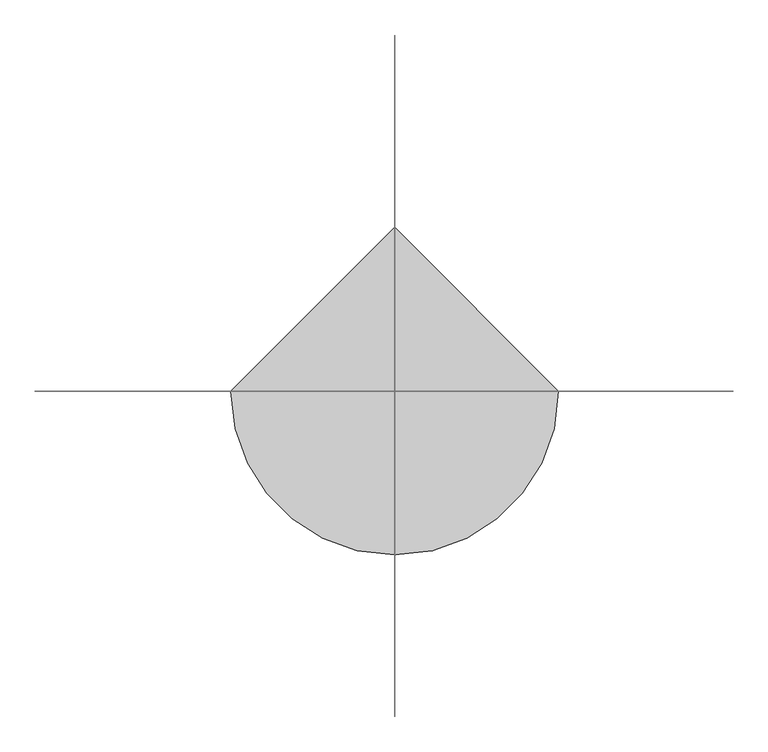
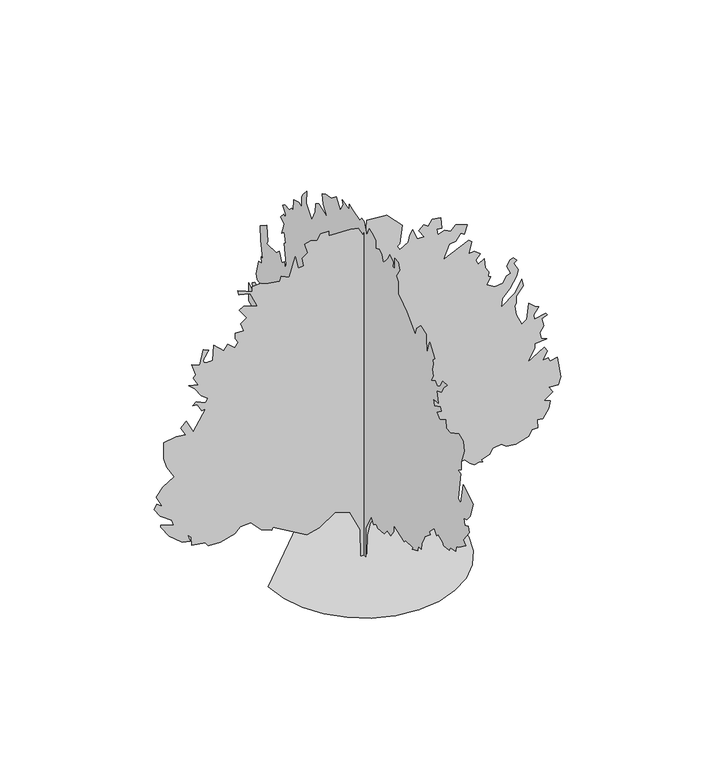
"""IFC4 building model written with IfcOpenShell, lengths in millimetres: proxy geometry, daphne 26070 : daphne 26070."""

import ifcopenshell
import ifcopenshell.guid

model = None  # the IFC model being written
_history = None  # IfcOwnerHistory: only IFC2X3 demands one
_inside = {}  # id of a spatial element -> (the spatial element, [elements in it])
_under = {}  # id of a project, library or spatial element -> (it, [spatial elements below it])
_declared = {}  # id of a project -> (the project, [libraries it declares])
_typed = {}  # id of a type object -> (the type object, [elements of that type])
_made_of = {}  # id of a material, layer set ... -> (it, [elements and type objects made of it])


def new_model(schema):
    """Start an empty IFC model of exactly this schema.

    Asked for "IFC4X3", IfcOpenShell would pick the latest addendum, in which some entities
    have other attributes; the version numbers below select the first issue.
    IFC2X3 requires an IfcOwnerHistory on every rooted entity: one is made here for all.
    """
    global model, _history
    if schema == "IFC4X3":
        model = ifcopenshell.file(schema_version=(4, 3, 0, 0))
    else:
        model = ifcopenshell.file(schema=schema)
    _inside.clear()
    _under.clear()
    _declared.clear()
    _typed.clear()
    _made_of.clear()
    _history = None
    if model.schema == "IFC2X3":
        org = make("IfcOrganization", Name="unknown")
        user = make(
            "IfcPersonAndOrganization",
            ThePerson=make("IfcPerson", FamilyName="unknown"),
            TheOrganization=org,
        )
        app = make(
            "IfcApplication",
            ApplicationDeveloper=org,
            Version="unknown",
            ApplicationFullName="unknown",
            ApplicationIdentifier="unknown",
        )
        _history = make(
            "IfcOwnerHistory",
            OwningUser=user,
            OwningApplication=app,
            ChangeAction="ADDED",
            CreationDate=0,
        )
    return model


def make(cls, **values):
    """One entity of the class cls with the attributes given. An attribute that is None is left unset."""
    return model.create_entity(
        cls, **{name: value for name, value in values.items() if value is not None}
    )


def rooted(cls, **values):
    """An entity with a GlobalId (a new one), such as an element, a storey or a relation."""
    return make(cls, GlobalId=ifcopenshell.guid.new(), OwnerHistory=_history, **values)


def si_unit(unit_type, name, prefix=None):
    """IfcSIUnit, for example si_unit("LENGTHUNIT", "METRE", prefix="MILLI")."""
    return make("IfcSIUnit", UnitType=unit_type, Prefix=prefix, Name=name)


def assignment(units):
    """IfcUnitAssignment: the units of a project."""
    return None if units is None else make("IfcUnitAssignment", Units=units)


def point(xyz):
    """IfcCartesianPoint."""
    return None if xyz is None else make("IfcCartesianPoint", Coordinates=xyz)


def direction(xyz):
    """IfcDirection."""
    return None if xyz is None else make("IfcDirection", DirectionRatios=xyz)


def frame(location, z_axis=None, x_axis=None):
    """IfcAxis2Placement3D, a coordinate frame: its origin and axes. An axis left out is left unset."""
    return make(
        "IfcAxis2Placement3D",
        Location=point(location),
        Axis=direction(z_axis),
        RefDirection=direction(x_axis),
    )


def origin():
    """The frame at (0, 0, 0) with its axes left unset."""
    return frame((0.0, 0.0, 0.0))


def place(relative_to, where):
    """IfcLocalPlacement: puts the frame where relative to a parent placement (None: the world)."""
    return make(
        "IfcLocalPlacement", PlacementRelTo=relative_to, RelativePlacement=where
    )


def context(
    kind, dimensions, precision=None, world=None, true_north=None, identifier=None
):
    """IfcGeometricRepresentationContext, for example the 3D "Model" context."""
    return make(
        "IfcGeometricRepresentationContext",
        ContextIdentifier=identifier,
        ContextType=kind,
        CoordinateSpaceDimension=dimensions,
        Precision=precision,
        WorldCoordinateSystem=world,
        TrueNorth=true_north,
    )


def project(units=None, contexts=None):
    """IfcProject with its units and contexts."""
    return rooted(
        "IfcProject",
        Name="project",
        RepresentationContexts=contexts,
        UnitsInContext=assignment(units),
    )


def spatial(cls, under=None, at=None, **own):
    """A site, building, storey or space (cls), placed at a placement, below another one or the project."""
    s = rooted(cls, ObjectPlacement=at, **own)
    if under is not None:
        _under.setdefault(under.id(), (under, []))[1].append(s)
    return s


def point_list(points):
    """IfcCartesianPointList2D or 3D."""
    cls = (
        "IfcCartesianPointList2D" if len(points[0]) == 2 else "IfcCartesianPointList3D"
    )
    return make(cls, CoordList=points)


def triangles(points, corners, closed=None, point_numbers=None):
    """IfcTriangulatedFaceSet: each triangle names its three corners, points numbered from 1."""
    return make(
        "IfcTriangulatedFaceSet",
        Coordinates=point_list(points),
        Closed=closed,
        CoordIndex=corners,
        PnIndex=point_numbers,
    )


def shape(context_of_items, identifier, shape_type, items):
    """IfcShapeRepresentation: the items that make up one representation, for example the "Body"."""
    return make(
        "IfcShapeRepresentation",
        ContextOfItems=context_of_items,
        RepresentationIdentifier=identifier,
        RepresentationType=shape_type,
        Items=items,
    )


def source(mapping_origin, context_of_items, identifier, shape_type, items):
    """IfcRepresentationMap: a shape defined once, which mapped items show again and again."""
    return make(
        "IfcRepresentationMap",
        MappingOrigin=mapping_origin,
        MappedRepresentation=shape(context_of_items, identifier, shape_type, items),
    )


def transform(
    local_origin,
    x_axis=None,
    y_axis=None,
    z_axis=None,
    scale=None,
    scale2=None,
    scale3=None,
    uniform=True,
):
    """IfcCartesianTransformationOperator3D, or its non-uniform kind. x_axis, y_axis, z_axis: its Axis1, 2, 3."""
    if uniform:
        return make(
            "IfcCartesianTransformationOperator3D",
            Axis1=direction(x_axis),
            Axis2=direction(y_axis),
            LocalOrigin=point(local_origin),
            Scale=scale,
            Axis3=direction(z_axis),
        )
    return make(
        "IfcCartesianTransformationOperator3DnonUniform",
        Axis1=direction(x_axis),
        Axis2=direction(y_axis),
        LocalOrigin=point(local_origin),
        Scale=scale,
        Axis3=direction(z_axis),
        Scale2=scale2,
        Scale3=scale3,
    )


def mapped(mapping_source, mapping_target):
    """IfcMappedItem: shows the shape of a source again, moved by a transform."""
    return make(
        "IfcMappedItem", MappingSource=mapping_source, MappingTarget=mapping_target
    )


def made_of(thing, what):
    """Note that an element or type object is made of a material, layer set ...; save() writes the relation."""
    if what is not None:
        _made_of.setdefault(what.id(), (what, []))[1].append(thing)
    return thing


def element(
    cls,
    number,
    at=None,
    inside=None,
    cuts=None,
    type_object=None,
    material=None,
    context=None,
    identifier="Body",
    shape_type=None,
    held_by="IfcProductDefinitionShape",
    body=None,
    shapes=None,
    **own,
):
    """One element of the class cls, such as IfcWall. Its Tag is "e" and its number.

    at: its placement. inside: the storey or other place that contains it. cuts: it is an
    opening in that element (IfcRelVoidsElement). A single representation is given by context,
    identifier, shape_type and body (its items); several are given by shapes. held_by: the class
    of the entity that holds the representations. save() writes the other relations.
    """
    e = rooted(cls, Tag="e%d" % number, ObjectPlacement=at, **own)
    if body is not None:
        shapes = [shape(context, identifier, shape_type, body)]
    if shapes is not None:
        e.Representation = make(held_by, Representations=shapes)
    if inside is not None:
        _inside.setdefault(inside.id(), (inside, []))[1].append(e)
    if cuts is not None:
        rooted(
            "IfcRelVoidsElement", RelatingBuildingElement=cuts, RelatedOpeningElement=e
        )
    if type_object is not None:
        _typed.setdefault(type_object.id(), (type_object, []))[1].append(e)
    return made_of(e, material)


def aggregate(whole, parts):
    """IfcRelAggregates: a whole, such as a stair, and the parts it consists of."""
    return rooted("IfcRelAggregates", RelatingObject=whole, RelatedObjects=parts)


def save(model, path):
    """Write the relations noted so far, then the file.

    IfcRelAggregates (storeys below a building ...), IfcRelContainedInSpatialStructure (elements
    in a storey), IfcRelDefinesByType, IfcRelAssociatesMaterial and IfcRelDeclares: one each for
    every whole, place, type object, material and project.
    """
    for whole, parts in _under.values():
        aggregate(whole, parts)
    for where, things in _inside.values():
        rooted(
            "IfcRelContainedInSpatialStructure",
            RelatedElements=things,
            RelatingStructure=where,
        )
    for kind, things in _typed.values():
        rooted("IfcRelDefinesByType", RelatedObjects=things, RelatingType=kind)
    for what, things in _made_of.values():
        rooted("IfcRelAssociatesMaterial", RelatedObjects=things, RelatingMaterial=what)
    for by, libraries in _declared.values():
        rooted("IfcRelDeclares", RelatingContext=by, RelatedDefinitions=libraries)
    model.write(path)


def entourage_7462b660(model_context):
    return source(origin(), model_context, "Body", "Tessellation", [
        triangles([(-9.4573925, -3.9e-06, 72.2348623), (-36.4693492, -6.1e-06, 128.8771626), (-74.629579, -5.2e-06, 141.2324949), (-113.9485589, -1.8e-06, 114.0498972), (-145.9624841, 1e-07, 106.0463523), (-234.001251, 8e-07, 158.0691489), (-236.002001, 1.4e-06, 150.0658583), (-264.0154255, 1.9e-06, 162.0709213), (-290.0250479, 1.3e-06, 190.0833467), (-318.0387268, 2.7e-06, 188.0823242), (-332.0443036, 4.1e-06, 174.0762387), (-368.4272936, 6.4e-06, 163.6409018), (-400.0731817, 7.6e-06, 166.0726938), (-408.0767266, 7.3e-06, 176.0772612), (-442.0924192, 8.5e-06, 182.0797836), (-444.0939686, 7.2e-06, 204.089414), (-452.0975135, 7.1e-06, 212.0929589), (-446.0929381, 7.9e-06, 194.0851191), (-466.1030903, 8.6e-06, 198.0868916), (-500.1187829, 8.4e-06, 226.0990444), (-522.1279046, 7.4e-06, 258.1124609), (-522.1279046, 7.1e-06, 264.1170363), (-488.1121757, 6.3e-06, 252.1104472), (-494.1142076, 5.6e-06, 268.117537), (-522.9229142, 5.6e-06, 288.9353979), (-538.1349944, 4.9e-06, 312.1357804), (-532.1304191, 3.9e-06, 324.1423513), (-518.1248423, 3.9e-06, 314.1372934), (-534.1319321, 2.8e-06, 344.14996), (-516.6084741, 8e-07, 365.2878413), (-486.7989927, -1.6e-06, 383.4742676), (-506.1208148, -2.7e-06, 416.1818642), (-514.1243597, -3.9e-06, 442.1940482), (-514.1243597, -6.5e-06, 486.2122553), (-482.1101801, -8.1e-06, 490.2153176), (-458.099509, -9.1e-06, 488.2138046), (-470.1035728, -9.9e-06, 510.2229263), (-456.097996, -1.13e-05, 524.2284668), (-438.0893932, -1e-05, 488.2138046), (-406.0752136, -1.45e-05, 540.2355566), (-416.0802715, -1.39e-05, 538.236587), (-428.0868788, -1.46e-05, 558.2441957), (-440.0909062, -1.42e-05, 560.2457088), (-430.0883918, -1.51e-05, 568.2492537), (-406.0752136, -1.54e-05, 556.2426827), (-401.4955876, -1.62e-05, 567.0275259), (-418.0817845, -1.63e-05, 580.2533175), (-434.0888743, -1.7e-05, 604.2639522), (-450.0959641, -1.72e-05, 618.2720724), (-426.0853294, -1.79e-05, 612.2674971), (-438.0893932, -1.87e-05, 634.2791622), (-432.0873613, -1.94e-05, 642.2826708), (-442.0924192, -2.07e-05, 672.2953737), (-422.0823034, -2.11e-05, 664.2917925), (-412.0797526, -2.38e-05, 702.308004), (-398.0716687, -2.41e-05, 696.3059721), (-400.6802304, -2.38e-05, 693.2783226), (-403.212634, -2.35e-05, 690.2023476), (-405.5926123, -2.32e-05, 687.0248526), (-407.7439708, -2.29e-05, 683.6948959), (-409.5930948, -2.26e-05, 680.1642975), (-411.0637536, -2.23e-05, 676.3821882), (-412.0797526, -2.21e-05, 672.2953737), (-411.9857903, -2.19e-05, 668.7317104), (-410.3525688, -2.18e-05, 666.420369), (-407.434106, -2.18e-05, 665.1452288), (-403.4920137, -2.2e-05, 664.7033226), (-398.7777666, -2.22e-05, 664.8861603), (-393.5530128, -2.25e-05, 665.485615), (-388.0691179, -2.28e-05, 666.2907984), (-386.0676049, -2.52e-05, 706.3085592), (-360.0554572, -2.49e-05, 682.2978882), (-350.0529064, -2.62e-05, 696.3059721), (-332.0443036, -2.6e-05, 680.2988823), (-322.0392457, -2.72e-05, 692.3029461), (-330.0427906, -2.76e-05, 704.3095533), (-330.0427906, -2.84e-05, 718.3150938), (-308.0336689, -2.94e-05, 718.3150938), (-316.0372138, -3.03e-05, 740.3242155), (-301.0029389, -3.16e-05, 751.5637184), (-320.0377327, -3.24e-05, 778.340427), (-308.0336689, -3.33e-05, 784.3424589), (-274.0179581, -3.42e-05, 774.3399445), (-292.0265791, -3.57e-05, 812.356156), (-320.9191106, -3.49e-05, 820.7254852), (-324.0407587, -3.54e-05, 832.3637283), (-304.0306247, -3.58e-05, 824.3602198), (-286.0245472, -3.62e-05, 816.3566385), (-286.0245472, -3.7e-05, 830.3647951), (-265.0619096, -3.8e-05, 832.6329706), (-252.0090908, -3.82e-05, 826.3616964), (-215.9931387, -3.95e-05, 820.3596645), (-211.9913662, -4.03e-05, 832.3637283), (-191.9827583, -4.06e-05, 822.3612139), (-175.9756504, -4.43e-05, 872.3814892), (-168.7203883, -4.27e-05, 839.3385933), (-153.9660381, -4.34e-05, 840.3673096), (-157.9678106, -4.45e-05, 862.3789747), (-143.9617251, -4.57e-05, 872.3814892), (-151.9650156, -4.69e-05, 898.3936369), (-135.9581802, -4.78e-05, 902.3941195), (-119.9513447, -4.83e-05, 898.3936369), (-109.9467864, -4.96e-05, 912.3991774), (-89.9381694, -5.05e-05, 912.3991774), (-89.9381694, -4.97e-05, 900.3951862), (-32.626833, -5.21e-05, 897.7739073), (-14.3439498, -5.26e-05, 893.5625364), (-1.8993678, -5.19e-05, 872.3814892), (6.1041838, -5.31e-05, 886.3895731), (8.105045, -5.45e-05, 908.3986948), (59.627565, -5.65e-05, 903.8140182), (99.4230465, -5.58e-05, 862.5999641), (92.1418776, -5.26e-05, 814.3577053), (86.1393461, -5.21e-05, 810.3546066), (92.1418776, -5.16e-05, 798.3505428), (114.1514989, -5.33e-05, 810.3546066), (118.1578496, -5.45e-05, 827.9416145), (126.1568253, -5.56e-05, 840.3673096), (138.1621427, -5.45e-05, 812.356156), (155.7905089, -5.52e-05, 811.8684677), (142.1639151, -5.58e-05, 832.3637283), (154.1689872, -5.71e-05, 844.3703356), (166.1743046, -5.71e-05, 836.3667543), (176.1785995, -5.85e-05, 852.3739168), (198.1884842, -5.92e-05, 848.3708181), (200.188998, -5.75e-05, 818.3581879), (188.1839168, -5.71e-05, 820.3596645), (190.1846849, -5.63e-05, 804.3525747), (208.1927972, -5.74e-05, 810.3546066), (224.199887, -5.76e-05, 802.3510981), (236.20495, -5.9e-05, 816.3566385), (265.7807247, -5.96e-05, 805.7293076), (258.2140718, -5.79e-05, 782.343453), (250.2110355, -5.79e-05, 788.3454849), (236.20495, -5.62e-05, 770.3369184), (220.1978602, -5.54e-05, 768.3379126), (204.1910248, -5.26e-05, 732.3207069), (270.2206608, -5.73e-05, 762.3333372), (278.2242057, -5.71e-05, 754.3298286), (270.2206608, -5.5e-05, 724.3171257), (284.2262195, -5.57e-05, 726.318675), (300.2333274, -5.57e-05, 714.3120678), (288.2267384, -5.43e-05, 700.3065273), (294.2312955, -5.39e-05, 688.3024635), (309.737998, -5.51e-05, 697.179756), (312.8444218, -5.37e-05, 671.3504459), (322.242431, -5.33e-05, 658.2872171), (320.240918, -5.25e-05, 646.283226), (326.2454933, -5.25e-05, 642.2801273), (316.2403991, -5.1e-05, 624.2741043), (337.7847236, -5.12e-05, 610.9797123), (358.2596729, -5.23e-05, 614.2690464), (368.2621874, -5.37e-05, 630.2761362), (378.0386619, -5.44e-05, 634.7135107), (368.2621874, -5.52e-05, 656.2882839), (376.2657323, -5.64e-05, 670.2938244), (384.2692772, -5.7e-05, 674.2943069), (394.2743714, -5.68e-05, 664.2917925), (386.2708265, -5.61e-05, 658.2872171), (398.1707179, -5.54e-05, 637.1290609), (394.2743714, -5.43e-05, 622.272555), (376.2657323, -5.17e-05, 592.2598884), (356.2581599, -4.97e-05, 572.2497725), (354.2566106, -4.83e-05, 550.2406508), (388.2723395, -5.13e-05, 576.2527986), (406.2783989, -5.4e-05, 608.2669782), (410.2814612, -5.3e-05, 588.2568624), (392.2728221, -5.09e-05, 566.2477407), (392.2728221, -4.98e-05, 548.2391015), (388.2723395, -4.93e-05, 542.2371059), (392.2728221, -4.79e-05, 516.2249219), (406.2783989, -4.67e-05, 486.2122553), (419.6692966, -4.79e-05, 495.1530613), (424.2870017, -5.05e-05, 536.235074), (440.2941278, -5.04e-05, 522.2294972), (450.2991858, -5.06e-05, 518.2264712), (437.047996, -4.89e-05, 500.1924339), (438.2925785, -4.83e-05, 488.2138046), (468.3077886, -4.99e-05, 494.2158002), (472.3083075, -4.97e-05, 488.2138046), (458.3027307, -4.88e-05, 482.2117727), (462.5902596, -4.78e-05, 462.3895815), (452.3006988, -4.64e-05, 446.1945308), (456.3012177, -4.56e-05, 430.187441), (470.3067581, -4.58e-05, 424.1854091), (440.2941278, -4.43e-05, 420.1849265), (440.2941278, -4.36e-05, 408.1783193), (420.2865191, -4.08e-05, 376.1641397), (464.3047626, -4.43e-05, 402.1762874), (472.3083075, -4.39e-05, 390.1697165), (460.3017002, -4.21e-05, 368.1605947), (474.3098205, -4.28e-05, 370.1621078), (478.3103394, -4.24e-05, 360.1570498), (498.3204552, -4.35e-05, 364.1600759), (506.3240001, -4.05e-05, 308.1352615), (500.3194247, -3.9e-05, 288.1251276), (476.3113335, -3.81e-05, 290.1266587), (486.3138843, -3.76e-05, 274.1195508), (464.3047626, -3.57e-05, 258.1124609), (480.3118524, -3.6e-05, 252.1104472), (476.3113335, -3.47e-05, 232.1015668), (460.3017002, -3.26e-05, 210.0919546), (446.2961234, -3.22e-05, 212.0929589), (448.2976727, -3.09e-05, 190.0833467), (432.2905829, -3.02e-05, 190.0833467), (424.2870017, -2.89e-05, 174.0762387), (391.7419679, -2.69e-05, 164.3614974), (366.2632178, -2.6e-05, 168.0737163), (354.2566106, -2.61e-05, 178.0780111), (332.2474889, -2.49e-05, 174.0762387), (323.8020015, -2.37e-05, 160.8723026), (302.2348404, -2.24e-05, 154.0673764), (306.2353412, -2.21e-05, 146.0640859), (298.2317963, -2.2e-05, 150.0658583), (284.2262195, -2.11e-05, 146.0640859), (272.2196304, -2.11e-05, 154.0673764), (260.2155848, -2.14e-05, 168.0737163), (240.2064682, -2.03e-05, 164.0719438), (236.8051496, -1.96e-05, 155.3752181), (196.1874799, -1.67e-05, 136.0595276), (196.1874799, -1.6e-05, 124.0544646), (162.1725321, -1.36e-05, 110.0481247), (162.1725321, -1.4e-05, 116.0509106), (138.1618883, -1.27e-05, 112.0491381), (106.7192036, -1.23e-05, 127.7984221), (83.214788, -1.13e-05, 128.4156446), (38.7434109, -8e-06, 104.983363), (17.3291135, -5.6e-06, 81.0641653), (9.1189377, -3.5e-06, 51.8726831), (8.1050195, -4e-07, 0.0), (-7.9020227, 3e-07, 7e-07), (-244.9072532, 0.0, 4.54e-05), (-238.4327937, -56.1165193, 4.18e-05), (-219.9933851, -107.6506239, 3.79e-05), (-191.0655541, -153.1257915, 3.39e-05), (-153.1257915, -191.0655541, 3e-05), (-107.6506239, -219.9933851, 2.63e-05), (-56.1165193, -238.4327937, 2.29e-05), (1.14e-05, -244.9072532, 2.01e-05), (56.1165193, -238.4327937, 1.8e-05), (107.6506239, -219.9933851, 5.12e-05), (153.1257915, -191.0655541, 5.1e-05), (191.0655541, -153.1257915, 5.16e-05), (219.9933851, -107.6506239, 1.87e-05), (238.4327937, -56.1165193, 2.09e-05), (244.9072532, 2.14e-05, 2.4e-05), (-3.16e-05, 244.9072532, 4.93e-05), (-1e-06, -8.7682648, 19.1210077), (-2.7e-06, -9.3654196, 78.8180451), (-6.1e-06, -33.2534526, 124.0544646), (-5.1e-06, -45.2590243, 110.0481247), (-5.2e-06, -55.2633328, 118.0516787), (-5.8e-06, -63.2666234, 112.0491381), (-6.9e-06, -91.2787853, 114.0498972), (-9e-06, -105.285116, 130.0569961), (-9.8e-06, -121.2919515, 126.0552236), (-9.6e-06, -133.2972779, 144.0630725), (-1.09e-05, -133.2972779, 162.0709213), (-1.16e-05, -181.318293, 146.0640859), (-1.37e-05, -187.3210879, 152.0666174), (-1.51e-05, -221.3357813, 154.0676308), (-1.31e-05, -215.3334951, 146.0640859), (-1.58e-05, -241.3446436, 158.0694032), (-1.53e-05, -243.3454117, 172.0754887), (-1.59e-05, -257.3504617, 172.0754887), (-1.75e-05, -259.3519928, 188.0825785), (-1.71e-05, -267.3555377, 204.089414), (-1.9e-05, -271.3585819, 214.0939814), (-1.92e-05, -297.3682044, 236.1036118), (-2.09e-05, -291.3661725, 240.1051299), (-2.09e-05, -315.3768253, 264.1170363), (-2.19e-05, -325.3818832, 250.1096791), (-2.19e-05, -331.3839151, 256.1134914), (-2.32e-05, -351.394031, 248.1086748), (-2.37e-05, -357.3960629, 242.1061342), (-2.46e-05, -381.4066976, 244.1069023), (-2.44e-05, -385.4072165, 254.1119602), (-2.53e-05, -409.4178512, 258.1124609), (-2.69e-05, -411.4193642, 272.1180377), (-2.71e-05, -423.423428, 278.1225949), (-2.96e-05, -455.4376076, 302.1332478), (-2.88e-05, -443.4335438, 310.1367745), (-3.05e-05, -469.4457278, 346.151473), (-3.18e-05, -465.4426655, 360.1570498), (-3.14e-05, -449.4355757, 354.1550179), (-3.05e-05, -445.4350931, 370.1621078), (-3.1e-05, -459.4406336, 374.1651701), (-3.29e-05, -474.5104623, 393.7968206), (-3.38e-05, -487.4517872, 434.1905033), (-3.29e-05, -443.4335438, 460.202651), (-3.07e-05, -433.4284859, 404.1778367), (-3e-05, -421.4244221, 408.1783193), (-3.36e-05, -431.6073034, 483.065209), (-3.29e-05, -419.4229091, 486.2122553), (-3.32e-05, -435.4299989, 496.2173495), (-3.43e-05, -435.4299989, 518.2264712), (-3.54e-05, -447.4340627, 554.2436769), (-3.64e-05, -443.4335438, 578.2543116), (-3.73e-05, -423.423428, 586.2578565), (-3.43e-05, -384.7290238, 566.6439737), (-3.35e-05, -367.3985773, 568.2492537), (-3.46e-05, -365.3996078, 590.2583754), (-3.2e-05, -339.38746, 574.2512856), (-3.09e-05, -325.3818832, 586.2578565), (-3.33e-05, -345.3894919, 600.2634333), (-3.26e-05, -341.388973, 610.2684912), (-3.2e-05, -313.375276, 596.2604073), (-3.12e-05, -309.3747934, 612.2674971), (-3.2e-05, -331.3839151, 614.2690464), (-3.26e-05, -324.6503509, 643.5704556), (-3.53e-05, -345.3894919, 652.2852579), (-3.49e-05, -357.3960629, 672.2953737), (-3.71e-05, -373.4031527, 688.3024635), (-3.62e-05, -351.394031, 686.3009142), (-3.44e-05, -341.388973, 668.2923477), (-3.42e-05, -327.3833962, 658.2897606), (-3.34e-05, -319.3798513, 668.2923477), (-3.31e-05, -301.3712485, 658.2897606), (-3.49e-05, -309.3747934, 674.2943069), (-3.4e-05, -305.3717311, 690.3013968), (-3.56e-05, -309.3747934, 706.3085592), (-3.5e-05, -307.3732804, 718.3150938), (-3.51e-05, -317.3783383, 726.318675), (-3.49e-05, -295.3692166, 758.3328547), (-3.52e-05, -289.3646595, 744.3272415), (-3.4e-05, -281.3610964, 716.3136171), (-3.58e-05, -279.3621268, 770.3369184), (-3.44e-05, -255.3514921, 778.340427), (-3.23e-05, -237.3428711, 760.334404), (-3.28e-05, -229.3393262, 740.3242155), (-3.11e-05, -209.330464, 760.334404), (-3.16e-05, -191.322606, 778.340427), (-3.05e-05, -177.3165205, 790.3470343), (-3.1e-05, -153.3061402, 804.3525747), (-3.17e-05, -153.3061402, 836.3667543), (-3.08e-05, -145.3025953, 848.3708181), (-3.26e-05, -161.3094307, 872.3814892), (-3.37e-05, -155.087445, 890.4942644), (-3.3e-05, -138.6373771, 891.588965), (-3.2e-05, -138.6373771, 863.4050749), (-3.17e-05, -129.7796238, 863.4050749), (-3.12e-05, -131.2962645, 876.3845152), (-3.22e-05, -115.28942, 886.3895731), (-3.04e-05, -107.2858751, 870.3824833), (-2.83e-05, -87.2770128, 848.3708181), (-2.94e-05, -81.2744813, 866.3794573), (-2.85e-05, -69.2691594, 874.3829659), (-2.82e-05, -53.2620651, 866.3794573), (-2.94e-05, -53.2620651, 888.388579), (-2.86e-05, -42.0070608, 894.8096987), (-2.75e-05, -25.2500576, 902.3966629), (-2.59e-05, -13.2446369, 878.3860645), (-2.63e-05, -3.2402807, 908.3986948), (-2.57e-05, 8.7649884, 910.4002441), (-2.58e-05, 16.768535, 900.3951862), (-2.39e-05, 50.7832783, 910.4002441), (-2.52e-05, 64.7893547, 914.4007267), (-2.37e-05, 64.7893547, 900.3951862), (-2.2e-05, 94.8025255, 908.3986948), (-2.26e-05, 90.8010074, 898.3936369), (-2.09e-05, 104.8068295, 874.3829659), (-2.11e-05, 122.8149417, 900.3951862), (-1.88e-05, 144.7590329, 883.3085838), (-1.79e-05, 169.2642141, 879.2750364), (-1.76e-05, 184.8420423, 870.3824833), (-1.68e-05, 179.1326343, 845.1882362), (-1.65e-05, 162.8324119, 820.3596645), (-1.63e-05, 200.8491321, 834.3652777), (-1.4e-05, 212.8544495, 826.3616964), (-1.49e-05, 216.8562219, 802.3510981), (-1.34e-05, 230.8623074, 772.3383951), (-1.32e-05, 254.871416, 802.3510981), (-1.4e-05, 252.8719378, 836.3667543), (-1.19e-05, 270.8810493, 816.3566385), (-1.21e-05, 276.8830812, 806.3541241), (-1.12e-05, 276.8830812, 778.340427), (-1.04e-05, 288.8871268, 784.3450024), (-9.7e-06, 310.8962485, 778.340427), (-8.7e-06, 314.8992745, 746.3262474), (-8.4e-06, 320.9013064, 748.3277967), (-6.3e-06, 330.9064007, 738.3227388), (-5.3e-06, 350.913973, 740.3242155), (-5.2e-06, 360.919031, 732.3207069), (-6.5e-06, 346.9134905, 716.3136171), (-4.7e-06, 348.9150035, 706.3085592), (-4.2e-06, 356.9185484, 710.3115852), (-4.3e-06, 368.9226122, 696.3059721), (-5.4e-06, 354.9170354, 684.2994375), (-4.1e-06, 364.9220933, 654.2867346), (-4.2e-06, 354.9170354, 662.2903158), (-3.5e-06, 346.9134905, 638.2796448), (-3.4e-06, 354.9170354, 632.2776129), (-1.8e-06, 344.9119411, 580.2533175), (-2.2e-06, 348.9150035, 568.2492537), (-1.3e-06, 354.9170354, 582.2548305), (-1.2e-06, 365.0364032, 574.0988966), (-1.8e-06, 376.9261571, 598.2619203), (4e-07, 388.932728, 586.2578565), (2.2e-06, 432.9509714, 584.2563435), (2.4e-06, 426.9489395, 594.2614014), (1e-07, 432.9509714, 634.2791622), (2.7e-06, 460.962125, 616.2705231), (3.1e-06, 458.9631191, 578.2543116), (5e-06, 448.9580612, 534.233561), (5.4e-06, 456.9616061, 534.233561), (4.5e-06, 453.2786187, 518.6607834), (5e-06, 466.966664, 516.2274653), (8e-06, 478.9707278, 474.2082278), (7.2e-06, 474.9702089, 460.202651), (6.5e-06, 460.962125, 458.201138), (7.6e-06, 458.9631191, 436.1920163), (9.3e-06, 484.9727597, 448.1960438), (9.4e-06, 495.8998544, 440.6471586), (1.04e-05, 490.9772987, 418.1833772), (9.7e-06, 512.9864204, 430.187441), (1.18e-05, 512.9864204, 380.167202), (9.6e-06, 476.9692148, 366.1616252), (1.23e-05, 498.9808436, 356.156531), (1.21e-05, 504.9828755, 346.151473), (1.23e-05, 478.9707278, 328.1428702), (1.17e-05, 462.963638, 330.1443832), (1.21e-05, 484.9727597, 316.1388064), (1.23e-05, 514.7745744, 340.233266), (1.35e-05, 520.9899653, 312.1357804), (1.38e-05, 508.9833944, 282.1231138), (1.52e-05, 530.9950596, 292.1281717), (1.67e-05, 532.7171565, 276.4538196), (1.52e-05, 513.8677983, 260.1292346), (1.52e-05, 504.9828755, 270.11905), (1.29e-05, 491.4116472, 278.5442443), (1.42e-05, 500.9798495, 300.1317166), (1.21e-05, 492.9763046, 308.1352615), (1.3e-05, 481.8053658, 291.1223283), (1.34e-05, 462.963638, 270.11905), (1.3e-05, 470.9671829, 252.1104472), (1.42e-05, 484.9727597, 266.1160058), (1.4e-05, 490.9772987, 256.1134914), (1.53e-05, 488.9757857, 238.1043617), (1.35e-05, 462.963638, 224.0982762), (1.52e-05, 472.9686959, 202.088664), (1.48e-05, 492.9763046, 222.0972719), (1.65e-05, 493.9364204, 210.9735868), (1.65e-05, 480.9722408, 176.0772612), (1.56e-05, 460.962125, 176.0772612), (1.7e-05, 462.963638, 156.0683989), (1.44e-05, 448.9580612, 160.0701714), (1.53e-05, 434.1422141, 145.3175835), (1.52e-05, 426.9489395, 150.0658583), (1.32e-05, 388.932728, 142.0623134), (1.26e-05, 374.9246078, 144.0630725), (1.31e-05, 378.9276701, 150.0658583), (1.21e-05, 350.913973, 156.0683989), (1.15e-05, 348.9150035, 144.0630725), (1.1e-05, 338.9099456, 142.0623134), (1.02e-05, 326.9033383, 136.0595276), (7.2e-06, 286.8856138, 158.0691489), (8.6e-06, 278.8845942, 148.0648449), (6.5e-06, 264.0916381, 164.6055958), (5.2e-06, 240.8666204, 158.0691489), (3.7e-06, 204.8506502, 158.0694032), (3.3e-06, 166.8341844, 138.060541), (3e-06, 170.8359568, 128.056237), (4.5e-06, 158.8306395, 124.0544646), (2.7e-06, 158.8306395, 132.0580095), (2e-06, 144.8243087, 130.0569961), (1.3e-06, 120.8141827, 138.060541), (-1e-06, 101.9528885, 154.2177488), (-2.5e-06, 36.7154756, 135.157575), (-1.1e-06, 12.638517, 93.3765678), (1.1e-06, 8.7649628, 3.52e-05), (3e-07, -9.2429405, 3.42e-05)], [[48, 49, 50], [94, 95, 96], [184, 185, 186], [212, 213, 214], [165, 166, 167], [165, 167, 168], [42, 43, 44], [52, 53, 54], [70, 71, 72], [42, 44, 45], [85, 86, 87], [84, 85, 87], [84, 87, 88], [41, 42, 45], [40, 41, 45], [173, 174, 175], [117, 118, 119], [17, 18, 19], [116, 117, 119], [144, 145, 146], [221, 222, 223], [21, 22, 23], [20, 21, 23], [132, 133, 134], [131, 132, 134], [130, 131, 134], [37, 38, 39], [36, 37, 39], [55, 56, 57], [164, 165, 168], [164, 168, 169], [164, 169, 170], [175, 176, 177], [173, 175, 177], [125, 126, 127], [179, 180, 181], [178, 179, 181], [173, 177, 178], [130, 134, 135], [130, 135, 136], [124, 125, 127], [123, 124, 127], [6, 7, 8], [26, 27, 28], [25, 26, 28], [80, 81, 82], [80, 82, 83], [157, 158, 159], [156, 157, 159], [155, 156, 159], [154, 155, 159], [154, 159, 160], [154, 160, 161], [92, 93, 94], [72, 73, 74], [203, 204, 205], [141, 142, 143], [193, 194, 195], [99, 100, 101], [55, 57, 58], [103, 104, 105], [76, 77, 78], [75, 76, 78], [109, 110, 111], [140, 141, 143], [99, 101, 102], [229, 230, 231], [229, 231, 1], [228, 229, 1], [188, 189, 190], [188, 190, 191], [197, 198, 199], [102, 103, 105], [148, 149, 150], [17, 19, 20], [17, 20, 23], [88, 89, 90], [154, 161, 162], [153, 154, 162], [152, 153, 162], [152, 162, 163], [151, 152, 163], [33, 34, 35], [228, 1, 2], [227, 228, 2], [83, 84, 88], [199, 200, 201], [47, 48, 50], [121, 122, 123], [120, 121, 123], [120, 123, 127], [120, 127, 128], [195, 196, 197], [193, 195, 197], [220, 221, 223], [191, 192, 193], [14, 15, 16], [78, 79, 80], [55, 58, 59], [54, 55, 59], [54, 59, 60], [54, 60, 61], [54, 61, 62], [54, 62, 63], [54, 63, 64], [54, 64, 65], [183, 184, 186], [129, 130, 136], [128, 129, 136], [137, 138, 139], [137, 139, 140], [83, 88, 90], [83, 90, 91], [83, 91, 92], [164, 170, 171], [28, 29, 30], [191, 193, 197], [188, 191, 197], [50, 51, 52], [24, 25, 28], [97, 98, 99], [109, 111, 112], [109, 112, 113], [109, 113, 114], [108, 109, 114], [128, 136, 137], [120, 128, 137], [201, 202, 203], [199, 201, 203], [178, 181, 182], [178, 182, 183], [33, 35, 36], [32, 33, 36], [31, 32, 36], [31, 36, 39], [119, 120, 137], [28, 30, 31], [52, 54, 65], [52, 65, 66], [50, 52, 66], [50, 66, 67], [50, 67, 68], [50, 68, 69], [116, 119, 137], [115, 116, 137], [172, 173, 178], [172, 178, 183], [172, 183, 186], [188, 197, 199], [24, 28, 31], [50, 69, 70], [214, 215, 216], [212, 214, 216], [212, 216, 217], [47, 50, 70], [46, 47, 70], [46, 70, 72], [46, 72, 74], [12, 13, 14], [205, 206, 207], [106, 107, 108], [137, 140, 143], [226, 227, 2], [146, 147, 148], [4, 5, 6], [3, 4, 6], [99, 102, 105], [97, 99, 105], [97, 105, 106], [97, 106, 108], [97, 108, 114], [97, 114, 115], [218, 219, 220], [137, 143, 144], [188, 199, 203], [188, 203, 205], [188, 205, 207], [188, 207, 208], [188, 208, 209], [188, 209, 210], [210, 211, 212], [210, 212, 217], [188, 210, 217], [188, 217, 218], [6, 8, 9], [78, 80, 83], [223, 224, 225], [220, 223, 225], [83, 92, 94], [11, 12, 14], [10, 11, 14], [10, 14, 16], [10, 16, 17], [10, 17, 23], [10, 23, 24], [10, 24, 31], [10, 31, 39], [9, 10, 39], [9, 39, 40], [6, 9, 40], [3, 6, 40], [3, 40, 45], [3, 45, 46], [3, 46, 74], [3, 74, 75], [3, 75, 78], [3, 78, 83], [3, 83, 94], [3, 94, 96], [3, 96, 97], [3, 97, 115], [3, 115, 137], [2, 3, 137], [226, 2, 137], [226, 137, 144], [226, 144, 146], [226, 146, 148], [226, 148, 150], [225, 226, 150], [220, 225, 150], [218, 220, 150], [188, 218, 150], [150, 151, 163], [150, 163, 164], [188, 150, 164], [188, 164, 171], [188, 171, 172], [188, 172, 186], [187, 188, 186], [246, 247, 232], [245, 246, 232], [245, 232, 233], [244, 245, 233], [244, 233, 234], [244, 234, 235], [243, 244, 235], [242, 243, 235], [242, 235, 236], [242, 236, 237], [242, 237, 238], [242, 238, 239], [242, 239, 240], [242, 240, 241], [261, 262, 263], [388, 389, 390], [372, 373, 374], [312, 313, 314], [440, 441, 442], [440, 442, 443], [312, 314, 315], [311, 312, 315], [358, 359, 360], [323, 324, 325], [414, 415, 416], [422, 423, 424], [301, 302, 303], [449, 450, 451], [400, 401, 402], [400, 402, 403], [399, 400, 403], [444, 445, 446], [311, 315, 316], [310, 311, 316], [289, 290, 291], [288, 289, 291], [287, 288, 291], [286, 287, 291], [280, 281, 282], [396, 397, 398], [322, 323, 325], [322, 325, 326], [462, 463, 464], [461, 462, 464], [425, 426, 427], [425, 427, 428], [425, 428, 429], [440, 443, 444], [268, 269, 270], [356, 357, 358], [394, 395, 396], [435, 436, 437], [435, 437, 438], [435, 438, 439], [425, 429, 430], [425, 430, 431], [424, 425, 431], [404, 405, 406], [372, 374, 375], [372, 375, 376], [456, 457, 458], [271, 272, 273], [371, 372, 376], [414, 416, 417], [308, 309, 310], [342, 343, 344], [341, 342, 344], [305, 306, 307], [304, 305, 307], [283, 284, 285], [282, 283, 285], [338, 339, 340], [337, 338, 340], [336, 337, 340], [361, 362, 363], [382, 383, 384], [381, 382, 384], [470, 471, 248], [469, 470, 248], [469, 248, 249], [469, 249, 250], [468, 469, 250], [386, 387, 388], [385, 386, 388], [399, 403, 404], [250, 251, 252], [350, 351, 352], [418, 419, 420], [417, 418, 420], [417, 420, 421], [321, 322, 326], [320, 321, 326], [292, 293, 294], [264, 265, 266], [316, 317, 318], [310, 316, 318], [308, 310, 318], [446, 447, 448], [424, 431, 432], [422, 424, 432], [422, 432, 433], [364, 365, 366], [277, 278, 279], [261, 263, 264], [255, 256, 257], [398, 399, 404], [326, 327, 328], [326, 328, 329], [326, 329, 330], [452, 453, 454], [396, 398, 404], [412, 413, 414], [411, 412, 414], [411, 414, 417], [377, 378, 379], [376, 377, 379], [336, 340, 341], [408, 409, 410], [341, 344, 345], [421, 422, 433], [421, 433, 434], [363, 364, 366], [363, 366, 367], [361, 363, 367], [407, 408, 410], [406, 407, 410], [391, 392, 393], [336, 341, 345], [255, 257, 258], [258, 259, 260], [379, 380, 381], [275, 276, 277], [274, 275, 277], [352, 353, 354], [352, 354, 355], [348, 349, 350], [348, 350, 352], [346, 347, 348], [345, 346, 348], [297, 298, 299], [297, 299, 300], [296, 297, 300], [294, 295, 296], [294, 296, 300], [294, 300, 301], [335, 336, 345], [334, 335, 345], [454, 455, 456], [452, 454, 456], [358, 360, 361], [367, 368, 369], [367, 369, 370], [286, 291, 292], [355, 356, 358], [448, 449, 451], [439, 440, 444], [396, 404, 406], [394, 396, 406], [394, 406, 410], [394, 410, 411], [371, 376, 379], [367, 370, 371], [294, 301, 303], [253, 254, 255], [252, 253, 255], [292, 294, 303], [318, 319, 320], [318, 320, 326], [318, 326, 330], [434, 435, 439], [352, 355, 358], [352, 358, 361], [352, 361, 367], [260, 261, 264], [411, 417, 421], [394, 411, 421], [252, 255, 258], [250, 252, 258], [348, 352, 367], [345, 348, 367], [334, 345, 367], [334, 367, 371], [333, 334, 371], [332, 333, 371], [331, 332, 371], [330, 331, 371], [318, 330, 371], [308, 318, 371], [307, 308, 371], [307, 371, 379], [307, 379, 381], [307, 381, 384], [307, 384, 385], [307, 385, 388], [307, 388, 390], [307, 390, 391], [307, 391, 393], [307, 393, 394], [307, 394, 421], [307, 421, 434], [307, 434, 439], [307, 439, 444], [307, 444, 446], [307, 446, 448], [307, 448, 451], [307, 451, 452], [307, 452, 456], [307, 456, 458], [307, 458, 459], [307, 459, 460], [307, 460, 461], [307, 461, 464], [307, 464, 465], [307, 465, 466], [307, 466, 467], [307, 467, 468], [307, 468, 250], [307, 250, 258], [304, 307, 258], [303, 304, 258], [292, 303, 258], [292, 258, 260], [273, 274, 277], [273, 277, 279], [271, 273, 279], [279, 280, 282], [271, 279, 282], [271, 282, 285], [271, 285, 286], [271, 286, 292], [271, 292, 260], [270, 271, 260], [268, 270, 260], [268, 260, 264], [268, 264, 266], [268, 266, 267]], closed=False),
    ])


if __name__ == "__main__":
    model = new_model("IFC4")
    model_context = context("Model", 3, world=origin())
    ifc_project = project(units=[si_unit("LENGTHUNIT", "METRE", prefix="MILLI")], contexts=[model_context])
    site = spatial("IfcSite", under=ifc_project)
    building = spatial("IfcBuilding", under=site)
    placement = place(None, origin())
    entourage_shape = entourage_7462b660(model_context)
    element("IfcBuildingElementProxy", 1, Name="daphne 26070 : daphne 26070", ObjectType="daphne 26070 : daphne 26070", at=placement, inside=building, context=model_context, shape_type="MappedRepresentation", body=[
        mapped(entourage_shape, transform((0.0, 0.0, 0.0), x_axis=(1.0, 0.0, 0.0), y_axis=(0.0, 1.0, 0.0), z_axis=(0.0, 0.0, 1.0))),
    ])
    save(model, "model.ifc")

# Revit data of these elements
# Type "daphne 26070 : daphne 26070"
#   built-in parameter 1005195 = "RPC-16-FUMB-EMQ0-U9RG-4000-ST1L-LVER-AU"
#   Height = 0
